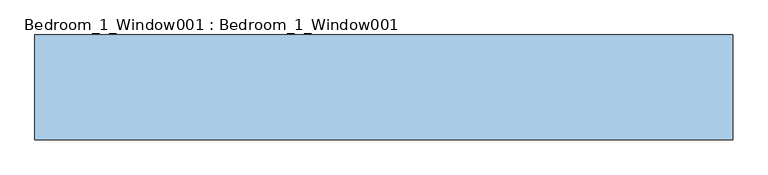
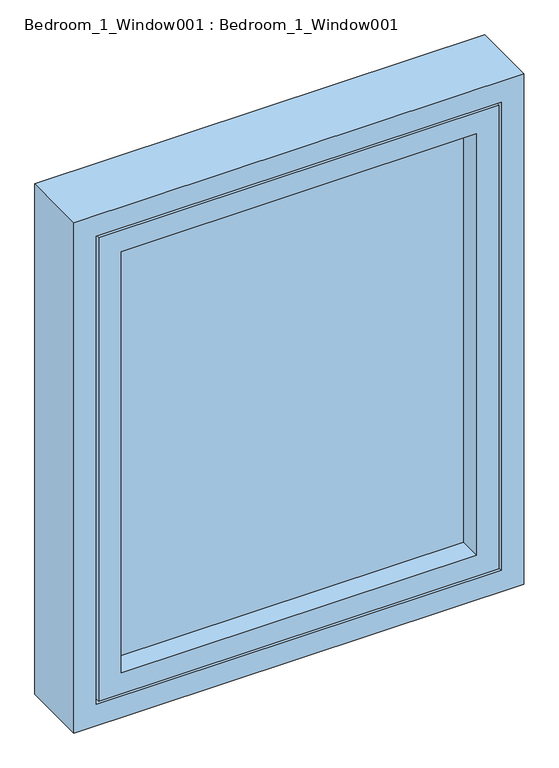
"""IFC4 building model written with IfcOpenShell, lengths in millimetres: window geometry, Bedroom_1_Window001 : Bedroom_1_Window001."""

from ifc_helpers import new_model, si_unit, frame, origin, place, context, project, spatial, polyline, outline, extrude, source, transform, mapped, element, save


def bedroom_1_window001_bedroom_1_window001_719b1152(model_context):
    return source(origin(), model_context, "Body", "SweptSolid", [
        extrude(outline(polyline([(2155.0, 405.0), (2945.0, 405.0), (2945.0, 395.0), (2155.0, 395.0), (2155.0, 405.0)])), frame((0.0, 0.0, 1355.0), z_axis=(0.0, 0.0, 1.0), x_axis=(1.0, 0.0, 0.0)), (0.0, 0.0, 1.0), 990.0),
        extrude(outline(polyline([(1305.0, 2995.0), (2395.0, 2995.0), (2395.0, 2105.0), (1305.0, 2105.0), (1305.0, 2995.0)]), holes=[polyline([(1355.0, 2155.0), (2345.0, 2155.0), (2345.0, 2945.0), (1355.0, 2945.0), (1355.0, 2155.0)])]), frame((0.0, 345.0, 0.0), z_axis=(0.0, 1.0, 0.0), x_axis=(0.0, 0.0, 1.0)), (0.0, 0.0, 1.0), 100.0),
        extrude(outline(polyline([(1250.0, 3050.0), (2450.0, 3050.0), (2450.0, 2050.0), (1250.0, 2050.0), (1250.0, 3050.0)]), holes=[polyline([(1300.0, 2100.0), (2400.0, 2100.0), (2400.0, 3000.0), (1300.0, 3000.0), (1300.0, 2100.0)])]), frame((0.0, 345.0, 0.0), z_axis=(0.0, 1.0, 0.0), x_axis=(0.0, 0.0, 1.0)), (0.0, 0.0, 1.0), 150.0),
    ])


if __name__ == "__main__":
    model = new_model("IFC4")
    model_context = context("Model", 3, world=origin())
    ifc_project = project(units=[si_unit("LENGTHUNIT", "METRE", prefix="MILLI")], contexts=[model_context])
    site = spatial("IfcSite", under=ifc_project)
    building = spatial("IfcBuilding", under=site)
    placement = place(None, origin())
    bedroom_1_window001_bedroom_1_window001_shape = bedroom_1_window001_bedroom_1_window001_719b1152(model_context)
    element("IfcWindow", 1, ObjectType="Bedroom_1_Window001 : Bedroom_1_Window001", at=placement, inside=building, context=model_context, shape_type="MappedRepresentation", body=[
        mapped(bedroom_1_window001_bedroom_1_window001_shape, transform((0.0, 0.0, 0.0), x_axis=(1.0, 0.0, 0.0), y_axis=(0.0, 1.0, 0.0), z_axis=(0.0, 0.0, 1.0))),
    ])
    save(model, "model.ifc")

# Revit data of these elements
# Type "Bedroom_1_Window001 : Bedroom_1_Window001"
#   Type Mark = "54"
#   NameOverride = "Bedroom_1_Window001"
# Element 1 (IfcWindow, "Bedroom_1_Window001 : Bedroom_1_Window001")
#   Materials on its faces: "IfcSurfaceStyle #392", "IfcSurfaceStyle #398"
# Materials
#   "IfcSurfaceStyle #392": class "Unassigned", colour RGB 204 204 204, transparency 0
#   "IfcSurfaceStyle #398": class "Unassigned", colour RGB 93 183 203, transparency 0.85
